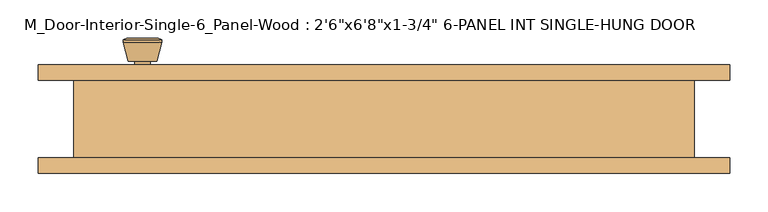
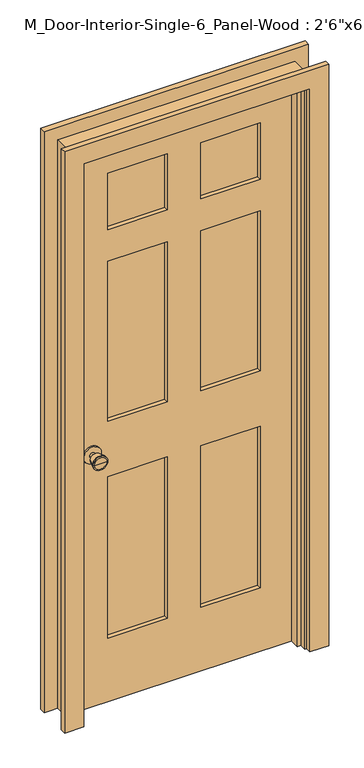
"""IFC4 building model written with IfcOpenShell, lengths in millimetres: door geometry."""

import ifcopenshell
import ifcopenshell.guid

model = None  # the IFC model being written
_history = None  # IfcOwnerHistory: only IFC2X3 demands one
_inside = {}  # id of a spatial element -> (the spatial element, [elements in it])
_under = {}  # id of a project, library or spatial element -> (it, [spatial elements below it])
_declared = {}  # id of a project -> (the project, [libraries it declares])
_typed = {}  # id of a type object -> (the type object, [elements of that type])
_made_of = {}  # id of a material, layer set ... -> (it, [elements and type objects made of it])


def new_model(schema):
    """Start an empty IFC model of exactly this schema.

    Asked for "IFC4X3", IfcOpenShell would pick the latest addendum, in which some entities
    have other attributes; the version numbers below select the first issue.
    IFC2X3 requires an IfcOwnerHistory on every rooted entity: one is made here for all.
    """
    global model, _history
    if schema == "IFC4X3":
        model = ifcopenshell.file(schema_version=(4, 3, 0, 0))
    else:
        model = ifcopenshell.file(schema=schema)
    _inside.clear()
    _under.clear()
    _declared.clear()
    _typed.clear()
    _made_of.clear()
    _history = None
    if model.schema == "IFC2X3":
        org = make("IfcOrganization", Name="unknown")
        user = make(
            "IfcPersonAndOrganization",
            ThePerson=make("IfcPerson", FamilyName="unknown"),
            TheOrganization=org,
        )
        app = make(
            "IfcApplication",
            ApplicationDeveloper=org,
            Version="unknown",
            ApplicationFullName="unknown",
            ApplicationIdentifier="unknown",
        )
        _history = make(
            "IfcOwnerHistory",
            OwningUser=user,
            OwningApplication=app,
            ChangeAction="ADDED",
            CreationDate=0,
        )
    return model


def make(cls, **values):
    """One entity of the class cls with the attributes given. An attribute that is None is left unset."""
    return model.create_entity(
        cls, **{name: value for name, value in values.items() if value is not None}
    )


def rooted(cls, **values):
    """An entity with a GlobalId (a new one), such as an element, a storey or a relation."""
    return make(cls, GlobalId=ifcopenshell.guid.new(), OwnerHistory=_history, **values)


def si_unit(unit_type, name, prefix=None):
    """IfcSIUnit, for example si_unit("LENGTHUNIT", "METRE", prefix="MILLI")."""
    return make("IfcSIUnit", UnitType=unit_type, Prefix=prefix, Name=name)


def assignment(units):
    """IfcUnitAssignment: the units of a project."""
    return None if units is None else make("IfcUnitAssignment", Units=units)


def point(xyz):
    """IfcCartesianPoint."""
    return None if xyz is None else make("IfcCartesianPoint", Coordinates=xyz)


def direction(xyz):
    """IfcDirection."""
    return None if xyz is None else make("IfcDirection", DirectionRatios=xyz)


def frame(location, z_axis=None, x_axis=None):
    """IfcAxis2Placement3D, a coordinate frame: its origin and axes. An axis left out is left unset."""
    return make(
        "IfcAxis2Placement3D",
        Location=point(location),
        Axis=direction(z_axis),
        RefDirection=direction(x_axis),
    )


def frame_2d(location, x_axis=None):
    """IfcAxis2Placement2D, a coordinate frame in the plane: its origin and x axis."""
    return make(
        "IfcAxis2Placement2D", Location=point(location), RefDirection=direction(x_axis)
    )


def origin():
    """The frame at (0, 0, 0) with its axes left unset."""
    return frame((0.0, 0.0, 0.0))


def place(relative_to, where):
    """IfcLocalPlacement: puts the frame where relative to a parent placement (None: the world)."""
    return make(
        "IfcLocalPlacement", PlacementRelTo=relative_to, RelativePlacement=where
    )


def context(
    kind, dimensions, precision=None, world=None, true_north=None, identifier=None
):
    """IfcGeometricRepresentationContext, for example the 3D "Model" context."""
    return make(
        "IfcGeometricRepresentationContext",
        ContextIdentifier=identifier,
        ContextType=kind,
        CoordinateSpaceDimension=dimensions,
        Precision=precision,
        WorldCoordinateSystem=world,
        TrueNorth=true_north,
    )


def project(units=None, contexts=None):
    """IfcProject with its units and contexts."""
    return rooted(
        "IfcProject",
        Name="project",
        RepresentationContexts=contexts,
        UnitsInContext=assignment(units),
    )


def spatial(cls, under=None, at=None, **own):
    """A site, building, storey or space (cls), placed at a placement, below another one or the project."""
    s = rooted(cls, ObjectPlacement=at, **own)
    if under is not None:
        _under.setdefault(under.id(), (under, []))[1].append(s)
    return s


def polyline(points):
    """IfcPolyline through the points."""
    return make("IfcPolyline", Points=[point(p) for p in points])


def circle_curve(where, radius):
    """IfcCircle in the frame where."""
    return make("IfcCircle", Position=where, Radius=radius)


def trimmed(basis, trim1, trim2, sense, master):
    """IfcTrimmedCurve: the piece of a basis curve between two trims."""
    return make(
        "IfcTrimmedCurve",
        BasisCurve=basis,
        Trim1=trim1,
        Trim2=trim2,
        SenseAgreement=sense,
        MasterRepresentation=master,
    )


def segment(curve, same_sense, transition):
    """IfcCompositeCurveSegment."""
    return make(
        "IfcCompositeCurveSegment",
        Transition=transition,
        SameSense=same_sense,
        ParentCurve=curve,
    )


def composite_curve(segments, self_intersect=None):
    """IfcCompositeCurve: segments joined end to end."""
    return make("IfcCompositeCurve", Segments=segments, SelfIntersect=self_intersect)


def outline(outer, holes=None, kind="AREA"):
    """IfcArbitraryClosedProfileDef: a profile drawn as a closed curve; with holes, ...WithVoids."""
    if holes is None:
        return make("IfcArbitraryClosedProfileDef", ProfileType=kind, OuterCurve=outer)
    return make(
        "IfcArbitraryProfileDefWithVoids",
        ProfileType=kind,
        OuterCurve=outer,
        InnerCurves=holes,
    )


def extrude(swept, where, along, depth):
    """IfcExtrudedAreaSolid: the profile swept, set in the frame where, extruded along a direction by depth."""
    return make(
        "IfcExtrudedAreaSolid",
        SweptArea=swept,
        Position=where,
        ExtrudedDirection=direction(along),
        Depth=depth,
    )


def faces_of(points, faces, orient=None, outer=None):
    """IfcFace entities. A face is a list of loops; a loop is a list of indices into points, from 0.

    orient and outer hold one flag for each loop. By default every Orientation is true, the
    first loop of a face is its IfcFaceOuterBound and the others are IfcFaceBound.
    """
    made = []
    for i, loops in enumerate(faces):
        bounds = []
        for j, loop in enumerate(loops):
            is_outer = j == 0 if outer is None else outer[i][j]
            bounds.append(
                make(
                    "IfcFaceOuterBound" if is_outer else "IfcFaceBound",
                    Bound=make("IfcPolyLoop", Polygon=[points[k] for k in loop]),
                    Orientation=True if orient is None else orient[i][j],
                )
            )
        made.append(make("IfcFace", Bounds=bounds))
    return made


def faceted_brep(points, faces, orient=None, outer=None, voids=None):
    """IfcFacetedBrep: a solid bounded by flat faces; with voids (closed shells), ...WithVoids."""
    shared = [point(p) for p in points]
    hull = make("IfcClosedShell", CfsFaces=faces_of(shared, faces, orient, outer))
    if voids is None:
        return make("IfcFacetedBrep", Outer=hull)
    return make(
        "IfcFacetedBrepWithVoids",
        Outer=hull,
        Voids=[
            make(cls, CfsFaces=faces_of(shared, fs, o, b)) for cls, fs, o, b in voids
        ],
    )


def shape(context_of_items, identifier, shape_type, items):
    """IfcShapeRepresentation: the items that make up one representation, for example the "Body"."""
    return make(
        "IfcShapeRepresentation",
        ContextOfItems=context_of_items,
        RepresentationIdentifier=identifier,
        RepresentationType=shape_type,
        Items=items,
    )


def source(mapping_origin, context_of_items, identifier, shape_type, items):
    """IfcRepresentationMap: a shape defined once, which mapped items show again and again."""
    return make(
        "IfcRepresentationMap",
        MappingOrigin=mapping_origin,
        MappedRepresentation=shape(context_of_items, identifier, shape_type, items),
    )


def transform(
    local_origin,
    x_axis=None,
    y_axis=None,
    z_axis=None,
    scale=None,
    scale2=None,
    scale3=None,
    uniform=True,
):
    """IfcCartesianTransformationOperator3D, or its non-uniform kind. x_axis, y_axis, z_axis: its Axis1, 2, 3."""
    if uniform:
        return make(
            "IfcCartesianTransformationOperator3D",
            Axis1=direction(x_axis),
            Axis2=direction(y_axis),
            LocalOrigin=point(local_origin),
            Scale=scale,
            Axis3=direction(z_axis),
        )
    return make(
        "IfcCartesianTransformationOperator3DnonUniform",
        Axis1=direction(x_axis),
        Axis2=direction(y_axis),
        LocalOrigin=point(local_origin),
        Scale=scale,
        Axis3=direction(z_axis),
        Scale2=scale2,
        Scale3=scale3,
    )


def mapped(mapping_source, mapping_target):
    """IfcMappedItem: shows the shape of a source again, moved by a transform."""
    return make(
        "IfcMappedItem", MappingSource=mapping_source, MappingTarget=mapping_target
    )


def made_of(thing, what):
    """Note that an element or type object is made of a material, layer set ...; save() writes the relation."""
    if what is not None:
        _made_of.setdefault(what.id(), (what, []))[1].append(thing)
    return thing


def element(
    cls,
    number,
    at=None,
    inside=None,
    cuts=None,
    type_object=None,
    material=None,
    context=None,
    identifier="Body",
    shape_type=None,
    held_by="IfcProductDefinitionShape",
    body=None,
    shapes=None,
    **own,
):
    """One element of the class cls, such as IfcWall. Its Tag is "e" and its number.

    at: its placement. inside: the storey or other place that contains it. cuts: it is an
    opening in that element (IfcRelVoidsElement). A single representation is given by context,
    identifier, shape_type and body (its items); several are given by shapes. held_by: the class
    of the entity that holds the representations. save() writes the other relations.
    """
    e = rooted(cls, Tag="e%d" % number, ObjectPlacement=at, **own)
    if body is not None:
        shapes = [shape(context, identifier, shape_type, body)]
    if shapes is not None:
        e.Representation = make(held_by, Representations=shapes)
    if inside is not None:
        _inside.setdefault(inside.id(), (inside, []))[1].append(e)
    if cuts is not None:
        rooted(
            "IfcRelVoidsElement", RelatingBuildingElement=cuts, RelatedOpeningElement=e
        )
    if type_object is not None:
        _typed.setdefault(type_object.id(), (type_object, []))[1].append(e)
    return made_of(e, material)


def aggregate(whole, parts):
    """IfcRelAggregates: a whole, such as a stair, and the parts it consists of."""
    return rooted("IfcRelAggregates", RelatingObject=whole, RelatedObjects=parts)


def save(model, path):
    """Write the relations noted so far, then the file.

    IfcRelAggregates (storeys below a building ...), IfcRelContainedInSpatialStructure (elements
    in a storey), IfcRelDefinesByType, IfcRelAssociatesMaterial and IfcRelDeclares: one each for
    every whole, place, type object, material and project.
    """
    for whole, parts in _under.values():
        aggregate(whole, parts)
    for where, things in _inside.values():
        rooted(
            "IfcRelContainedInSpatialStructure",
            RelatedElements=things,
            RelatingStructure=where,
        )
    for kind, things in _typed.values():
        rooted("IfcRelDefinesByType", RelatedObjects=things, RelatingType=kind)
    for what, things in _made_of.values():
        rooted("IfcRelAssociatesMaterial", RelatedObjects=things, RelatingMaterial=what)
    for by, libraries in _declared.values():
        rooted("IfcRelDeclares", RelatingContext=by, RelatedDefinitions=libraries)
    model.write(path)


def plane_surface(at):
    """IfcPlane: the flat surface through the origin of the frame at, square to its z axis."""
    return make("IfcPlane", Position=at)


def cylinder_surface(at, radius):
    """IfcCylindricalSurface: all points at the distance radius from the z axis of the frame at."""
    return make("IfcCylindricalSurface", Position=at, Radius=radius)


def revolved_surface(curve, axis_point, axis_direction):
    """IfcSurfaceOfRevolution: the curve turned about the line through axis_point along axis_direction."""
    return make(
        "IfcSurfaceOfRevolution",
        SweptCurve=make("IfcArbitraryOpenProfileDef", ProfileType="CURVE", Curve=curve),
        AxisPosition=make("IfcAxis1Placement", Location=point(axis_point), Axis=direction(axis_direction)),
    )


def advanced_brep(points, edges, surfaces, faces):
    """IfcAdvancedBrep: a solid bounded by faces that lie on surfaces and meet in shared edges.

    An edge is (start, end): straight between two places in points (the first is 0);
    or (start, end, curve); or (start, end, curve, False) where it runs against its curve.
    A face is (place in surfaces, loops), or (place, loops, False) where it looks against
    its surface's normal. A loop lists edges by number (the first is 1), with a minus sign
    where the edge is run from its end to its start. The first loop is the outer one.
    """
    corners = [point(p) for p in points]
    vertices = [make("IfcVertexPoint", VertexGeometry=c) for c in corners]
    made = []
    for start, end, *more in edges:
        made.append(
            make(
                "IfcEdgeCurve",
                EdgeStart=vertices[start],
                EdgeEnd=vertices[end],
                EdgeGeometry=more[0] if more else make("IfcPolyline", Points=[corners[start], corners[end]]),
                SameSense=more[1] if len(more) > 1 else True,
            )
        )
    hull = []
    for where, loops, *sense in faces:
        bounds = []
        for j, loop in enumerate(loops):
            ring = [make("IfcOrientedEdge", EdgeElement=made[abs(k) - 1], Orientation=k > 0) for k in loop]
            bounds.append(
                make(
                    "IfcFaceOuterBound" if j == 0 else "IfcFaceBound",
                    Bound=make("IfcEdgeLoop", EdgeList=ring),
                    Orientation=True,
                )
            )
        hull.append(make("IfcAdvancedFace", Bounds=bounds, FaceSurface=surfaces[where], SameSense=sense[0] if sense else True))
    return make("IfcAdvancedBrep", Outer=make("IfcClosedShell", CfsFaces=hull))


def door_beb2e203(model_context):
    return source(origin(), model_context, "Body", "SolidModel", [
        advanced_brep(
        [(-316.0, -2.825, 914.4), (-306.0, -2.825, 914.4), (-326.0, -2.825, 914.4), (-295.5241324, -51.825, 914.4), (-316.0, -51.825, 914.4), (-336.4758676, -51.825, 914.4), (-291.0, -49.9971319, 914.4), (-341.0, -49.9971319, 914.4), (-291.0, -46.5334537, 914.4), (-341.0, -46.5334537, 914.4), (-297.363764, -21.825, 914.4), (-334.636236, -21.825, 914.4), (-306.0, -21.825, 914.4), (-326.0, -21.825, 914.4)],
        [
            (0, 1),
            (1, 2, circle_curve(frame((-316.0, -2.825, 914.4), z_axis=(0.0, 1.0, 0.0), x_axis=(-1.0, 0.0, 0.0)), 10.0)),
            (2, 0),
            (2, 1, circle_curve(frame((-316.0, -2.825, 914.4), z_axis=(0.0, 1.0, 0.0), x_axis=(-1.0, 0.0, 0.0)), 10.0)),
            (3, 4),
            (4, 5),
            (5, 3, circle_curve(frame((-316.0, -51.825, 914.4), z_axis=(0.0, -1.0, 0.0), x_axis=(-1.0, 0.0, 0.0)), 20.4758676)),
            (3, 5, circle_curve(frame((-316.0, -51.825, 914.4), z_axis=(0.0, -1.0, 0.0), x_axis=(-1.0, 0.0, 0.0)), 20.4758676)),
            (6, 3),
            (5, 7),
            (7, 6, circle_curve(frame((-316.0, -49.9971319, 914.4), z_axis=(0.0, -1.0, 0.0), x_axis=(-1.0, 0.0, 0.0)), 25.0)),
            (6, 7, circle_curve(frame((-316.0, -49.9971319, 914.4), z_axis=(0.0, -1.0, 0.0), x_axis=(-1.0, 0.0, 0.0)), 25.0)),
            (8, 6),
            (7, 9),
            (9, 8, circle_curve(frame((-316.0, -46.5334537, 914.4), z_axis=(0.0, -1.0, 0.0), x_axis=(-1.0, 0.0, 0.0)), 25.0)),
            (8, 9, circle_curve(frame((-316.0, -46.5334537, 914.4), z_axis=(0.0, -1.0, 0.0), x_axis=(-1.0, 0.0, 0.0)), 25.0)),
            (10, 8),
            (9, 11),
            (11, 10, circle_curve(frame((-316.0, -21.825, 914.4), z_axis=(0.0, -1.0, 0.0), x_axis=(-1.0, 0.0, 0.0)), 18.636236)),
            (10, 11, circle_curve(frame((-316.0, -21.825, 914.4), z_axis=(0.0, -1.0, 0.0), x_axis=(-1.0, 0.0, 0.0)), 18.636236)),
            (12, 10),
            (11, 13),
            (13, 12, circle_curve(frame((-316.0, -21.825, 914.4), z_axis=(0.0, -1.0, 0.0), x_axis=(-1.0, 0.0, 0.0)), 10.0)),
            (12, 13, circle_curve(frame((-316.0, -21.825, 914.4), z_axis=(0.0, -1.0, 0.0), x_axis=(-1.0, 0.0, 0.0)), 10.0)),
            (1, 12),
            (13, 2),
        ],
        [
            plane_surface(frame((-316.0, -2.825, 914.4), z_axis=(0.0, 1.0, 0.0), x_axis=(-1.0, 0.0, 0.0))),
            plane_surface(frame((-316.0, -51.825, 914.4), z_axis=(0.0, -1.0, 0.0), x_axis=(-1.0, 0.0, 0.0))),
            revolved_surface(polyline([(-336.4758676, -51.825, 914.4), (-341.0, -49.9971319, 914.4)]), (-316.0, -2.825, 914.4), (0.0, 1.0, 0.0)),
            cylinder_surface(frame((-316.0, -2.825, 914.4), z_axis=(0.0, 1.0, 0.0), x_axis=(-1.0, 0.0, 0.0)), 25.0),
            revolved_surface(polyline([(-341.0, -46.5334537, 914.4), (-334.636236, -21.825, 914.4)]), (-316.0, -2.825, 914.4), (0.0, 1.0, 0.0)),
            plane_surface(frame((-316.0, -21.825, 914.4), z_axis=(0.0, 1.0, 0.0), x_axis=(-1.0, 0.0, 0.0))),
            cylinder_surface(frame((-316.0, -2.825, 914.4), z_axis=(0.0, 1.0, 0.0), x_axis=(-1.0, 0.0, 0.0)), 10.0),
        ],
        [
            (0, [[1, 2, 3]]),
            (0, [[-3, 4, -1]]),
            (1, [[5, 6, 7]]),
            (1, [[-6, -5, 8]]),
            (2, [[9, -7, 10, 11]]),
            (2, [[-10, -8, -9, 12]]),
            (3, [[13, -11, 14, 15]]),
            (3, [[-14, -12, -13, 16]]),
            (4, [[17, -15, 18, 19]]),
            (4, [[-18, -16, -17, 20]]),
            (5, [[21, -19, 22, 23]]),
            (5, [[-22, -20, -21, 24]]),
            (6, [[25, -23, 26, -2]]),
            (6, [[-26, -24, -25, -4]]),
        ],
    ),
        extrude(outline(composite_curve([segment(trimmed(circle_curve(frame_2d((914.4, -316.0)), 30.0), [point((914.4, -346.0))], [point((914.4, -286.0))], False, "CARTESIAN"), True, "CONTINUOUS"), segment(trimmed(circle_curve(frame_2d((914.4, -316.0)), 30.0), [point((914.4, -286.0))], [point((914.4, -346.0))], False, "CARTESIAN"), True, "CONTINUOUS")], self_intersect=False)), frame((0.0, -2.825, 0.0), z_axis=(0.0, 1.0, 0.0), x_axis=(0.0, 0.0, 1.0)), (0.0, 0.0, 1.0), 6.0),
        advanced_brep(
        [(-316.0, 53.625, 914.4), (-326.0, 53.625, 914.4), (-306.0, 53.625, 914.4), (-295.5241324, 102.625, 914.4), (-336.4758676, 102.625, 914.4), (-316.0, 102.625, 914.4), (-291.0, 100.7971319, 914.4), (-341.0, 100.7971319, 914.4), (-291.0, 97.3334537, 914.4), (-341.0, 97.3334537, 914.4), (-297.363764, 72.625, 914.4), (-334.636236, 72.625, 914.4), (-306.0, 72.625, 914.4), (-326.0, 72.625, 914.4)],
        [
            (0, 1),
            (1, 2, circle_curve(frame((-316.0, 53.625, 914.4), z_axis=(0.0, -1.0, 0.0), x_axis=(-1.0, 0.0, 0.0)), 10.0)),
            (2, 0),
            (2, 1, circle_curve(frame((-316.0, 53.625, 914.4), z_axis=(0.0, -1.0, 0.0), x_axis=(-1.0, 0.0, 0.0)), 10.0)),
            (3, 4, circle_curve(frame((-316.0, 102.625, 914.4), z_axis=(0.0, 1.0, 0.0), x_axis=(-1.0, 0.0, 0.0)), 20.4758676)),
            (4, 5),
            (5, 3),
            (4, 3, circle_curve(frame((-316.0, 102.625, 914.4), z_axis=(0.0, 1.0, 0.0), x_axis=(-1.0, 0.0, 0.0)), 20.4758676)),
            (6, 7, circle_curve(frame((-316.0, 100.7971319, 914.4), z_axis=(0.0, 1.0, 0.0), x_axis=(-1.0, 0.0, 0.0)), 25.0)),
            (7, 4),
            (3, 6),
            (7, 6, circle_curve(frame((-316.0, 100.7971319, 914.4), z_axis=(0.0, 1.0, 0.0), x_axis=(-1.0, 0.0, 0.0)), 25.0)),
            (8, 9, circle_curve(frame((-316.0, 97.3334537, 914.4), z_axis=(0.0, 1.0, 0.0), x_axis=(-1.0, 0.0, 0.0)), 25.0)),
            (9, 7),
            (6, 8),
            (9, 8, circle_curve(frame((-316.0, 97.3334537, 914.4), z_axis=(0.0, 1.0, 0.0), x_axis=(-1.0, 0.0, 0.0)), 25.0)),
            (10, 11, circle_curve(frame((-316.0, 72.625, 914.4), z_axis=(0.0, 1.0, 0.0), x_axis=(-1.0, 0.0, 0.0)), 18.636236)),
            (11, 9),
            (8, 10),
            (11, 10, circle_curve(frame((-316.0, 72.625, 914.4), z_axis=(0.0, 1.0, 0.0), x_axis=(-1.0, 0.0, 0.0)), 18.636236)),
            (12, 13, circle_curve(frame((-316.0, 72.625, 914.4), z_axis=(0.0, 1.0, 0.0), x_axis=(-1.0, 0.0, 0.0)), 10.0)),
            (13, 11),
            (10, 12),
            (13, 12, circle_curve(frame((-316.0, 72.625, 914.4), z_axis=(0.0, 1.0, 0.0), x_axis=(-1.0, 0.0, 0.0)), 10.0)),
            (1, 13),
            (12, 2),
        ],
        [
            plane_surface(frame((-316.0, 53.625, 914.4), z_axis=(0.0, -1.0, 0.0), x_axis=(-1.0, 0.0, 0.0))),
            plane_surface(frame((-316.0, 102.625, 914.4), z_axis=(0.0, 1.0, 0.0), x_axis=(-1.0, 0.0, 0.0))),
            revolved_surface(polyline([(-336.4758676, 102.625, 914.4), (-341.0, 100.7971319, 914.4)]), (-316.0, 53.625, 914.4), (0.0, -1.0, 0.0)),
            cylinder_surface(frame((-316.0, 53.625, 914.4), z_axis=(0.0, -1.0, 0.0), x_axis=(-1.0, 0.0, 0.0)), 25.0),
            revolved_surface(polyline([(-341.0, 97.3334537, 914.4), (-334.636236, 72.625, 914.4)]), (-316.0, 53.625, 914.4), (0.0, -1.0, 0.0)),
            plane_surface(frame((-316.0, 72.625, 914.4), z_axis=(0.0, -1.0, 0.0), x_axis=(-1.0, 0.0, 0.0))),
            cylinder_surface(frame((-316.0, 53.625, 914.4), z_axis=(0.0, -1.0, 0.0), x_axis=(-1.0, 0.0, 0.0)), 10.0),
        ],
        [
            (0, [[1, 2, 3]]),
            (0, [[-3, 4, -1]]),
            (1, [[5, 6, 7]]),
            (1, [[8, -7, -6]]),
            (2, [[9, 10, -5, 11]]),
            (2, [[12, -11, -8, -10]]),
            (3, [[13, 14, -9, 15]]),
            (3, [[16, -15, -12, -14]]),
            (4, [[17, 18, -13, 19]]),
            (4, [[20, -19, -16, -18]]),
            (5, [[21, 22, -17, 23]]),
            (5, [[24, -23, -20, -22]]),
            (6, [[-2, 25, -21, 26]]),
            (6, [[-4, -26, -24, -25]]),
        ],
    ),
        extrude(outline(composite_curve([segment(trimmed(circle_curve(frame_2d((914.4, -316.0)), 30.0), [point((914.4, -346.0))], [point((914.4, -286.0))], False, "CARTESIAN"), True, "CONTINUOUS"), segment(trimmed(circle_curve(frame_2d((914.4, -316.0)), 30.0), [point((914.4, -286.0))], [point((914.4, -346.0))], False, "CARTESIAN"), True, "CONTINUOUS")], self_intersect=False)), frame((0.0, 47.625, 0.0), z_axis=(0.0, 1.0, 0.0), x_axis=(0.0, 0.0, 1.0)), (0.0, 0.0, 1.0), 6.0),
        extrude(outline(polyline([(261.0, 17.9916667), (57.5, 17.9916667), (57.5, 32.8083333), (261.0, 32.8083333), (261.0, 17.9916667)])), frame((0.0, 0.0, 1708.5), z_axis=(0.0, 0.0, 1.0), x_axis=(1.0, 0.0, 0.0)), (0.0, 0.0, 1.0), 203.5),
        extrude(outline(polyline([(261.0, 17.9916667), (57.5, 17.9916667), (57.5, 32.8083333), (261.0, 32.8083333), (261.0, 17.9916667)])), frame((0.0, 0.0, 1014.4), z_axis=(0.0, 0.0, 1.0), x_axis=(1.0, 0.0, 0.0)), (0.0, 0.0, 1.0), 579.1),
        extrude(outline(polyline([(-57.5, 17.9916667), (-261.0, 17.9916667), (-261.0, 32.8083333), (-57.5, 32.8083333), (-57.5, 17.9916667)])), frame((0.0, 0.0, 1014.4), z_axis=(0.0, 0.0, 1.0), x_axis=(1.0, 0.0, 0.0)), (0.0, 0.0, 1.0), 579.1),
        extrude(outline(polyline([(-57.5, 17.9916667), (-261.0, 17.9916667), (-261.0, 32.8083333), (-57.5, 32.8083333), (-57.5, 17.9916667)])), frame((0.0, 0.0, 1708.5), z_axis=(0.0, 0.0, 1.0), x_axis=(1.0, 0.0, 0.0)), (0.0, 0.0, 1.0), 203.5),
        extrude(outline(polyline([(261.0, 17.9916667), (57.5, 17.9916667), (57.5, 32.8083333), (261.0, 32.8083333), (261.0, 17.9916667)])), frame((0.0, 0.0, 230.0), z_axis=(0.0, 0.0, 1.0), x_axis=(1.0, 0.0, 0.0)), (0.0, 0.0, 1.0), 584.4),
        extrude(outline(polyline([(-57.5, 17.9916667), (-261.0, 17.9916667), (-261.0, 32.8083333), (-57.5, 32.8083333), (-57.5, 17.9916667)])), frame((0.0, 0.0, 230.0), z_axis=(0.0, 0.0, 1.0), x_axis=(1.0, 0.0, 0.0)), (0.0, 0.0, 1.0), 584.4),
        extrude(outline(polyline([(2032.0, -381.0), (0.0, -381.0), (0.0, 381.0), (2032.0, 381.0), (2032.0, -381.0)]), holes=[polyline([(1912.0, 57.5), (1912.0, 261.0), (1708.5, 261.0), (1708.5, 57.5), (1912.0, 57.5)]), polyline([(1593.5, 261.0), (1014.4, 261.0), (1014.4, 57.5), (1593.5, 57.5), (1593.5, 261.0)]), polyline([(1014.4, -57.5), (1014.4, -261.0), (1593.5, -261.0), (1593.5, -57.5), (1014.4, -57.5)]), polyline([(1708.5, -261.0), (1912.0, -261.0), (1912.0, -57.5), (1708.5, -57.5), (1708.5, -261.0)]), polyline([(814.4, 57.5), (814.4, 261.0), (230.0, 261.0), (230.0, 57.5), (814.4, 57.5)]), polyline([(230.0, -57.5), (230.0, -261.0), (814.4, -261.0), (814.4, -57.5), (230.0, -57.5)])]), frame((0.0, 3.175, 0.0), z_axis=(0.0, 1.0, 0.0), x_axis=(0.0, 0.0, 1.0)), (0.0, 0.0, 1.0), 44.45),
        faceted_brep([(406.0, 47.625, 0.0), (406.0, -53.975, 0.0), (381.0, -53.975, 0.0), (381.0, -31.75, 0.0), (368.3, -31.75, 0.0), (368.3, 3.175, 0.0), (381.0, 3.175, 0.0), (381.0, 47.625, 0.0), (406.0, 47.625, 2057.0), (406.0, -53.975, 2057.0), (-406.0, -53.975, 2057.0), (-406.0, -53.975, 0.0), (-381.0, -53.975, 0.0), (-381.0, -53.975, 2032.0), (381.0, -53.975, 2032.0), (381.0, -31.75, 2032.0), (-381.0, -31.75, 2032.0), (-381.0, -31.75, 0.0), (-368.3, -31.75, 0.0), (-368.3, -31.75, 2019.3), (368.3, -31.75, 2019.3), (368.3, 3.175, 2019.3), (-368.3, 3.175, 2019.3), (-368.3, 3.175, 0.0), (-381.0, 3.175, 0.0), (-381.0, 3.175, 2032.0), (381.0, 3.175, 2032.0), (381.0, 47.625, 2032.0), (-381.0, 47.625, 2032.0), (-381.0, 47.625, 0.0), (-406.0, 47.625, 0.0), (-406.0, 47.625, 2057.0)], [[[0, 1, 2, 3, 4, 5, 6, 7]], [[1, 0, 8, 9]], [[2, 1, 9, 10, 11, 12, 13, 14]], [[3, 2, 14, 15]], [[4, 3, 15, 16, 17, 18, 19, 20]], [[5, 4, 20, 21]], [[6, 5, 21, 22, 23, 24, 25, 26]], [[7, 6, 26, 27]], [[0, 7, 27, 28, 29, 30, 31, 8]], [[9, 8, 31, 10]], [[15, 14, 13, 16]], [[21, 20, 19, 22]], [[27, 26, 25, 28]], [[30, 29, 24, 23, 18, 17, 12, 11]], [[10, 31, 30, 11]], [[16, 13, 12, 17]], [[22, 19, 18, 23]], [[28, 25, 24, 29]]]),
        extrude(outline(polyline([(0.0, 387.35), (0.0, 452.35), (2103.35, 452.35), (2103.35, -452.35), (0.0, -452.35), (0.0, -387.35), (2038.35, -387.35), (2038.35, 387.35), (0.0, 387.35)])), frame((0.0, -73.975, 0.0), z_axis=(0.0, 1.0, 0.0), x_axis=(0.0, 0.0, 1.0)), (0.0, 0.0, 1.0), 20.0),
        extrude(outline(polyline([(0.0, 387.35), (0.0, 452.35), (2103.35, 452.35), (2103.35, -452.35), (0.0, -452.35), (0.0, -387.35), (2038.35, -387.35), (2038.35, 387.35), (0.0, 387.35)])), frame((0.0, 47.625, 0.0), z_axis=(0.0, 1.0, 0.0), x_axis=(0.0, 0.0, 1.0)), (0.0, 0.0, 1.0), 20.0),
    ])


if __name__ == "__main__":
    model = new_model("IFC4")
    model_context = context("Model", 3, world=origin())
    ifc_project = project(units=[si_unit("LENGTHUNIT", "METRE", prefix="MILLI")], contexts=[model_context])
    site = spatial("IfcSite", under=ifc_project)
    building = spatial("IfcBuilding", under=site)
    placement = place(None, origin())
    door_shape = door_beb2e203(model_context)
    element("IfcDoor", 1, ObjectType="M_Door-Interior-Single-6_Panel-Wood : 2'6\"x6'8\"x1-3/4\" 6-PANEL INT SINGLE-HUNG DOOR", at=placement, inside=building, context=model_context, shape_type="MappedRepresentation", body=[
        mapped(door_shape, transform((0.0, 0.0, 0.0), x_axis=(1.0, 0.0, 0.0), y_axis=(0.0, 1.0, 0.0), z_axis=(0.0, 0.0, 1.0))),
    ])
    save(model, "model.ifc")

# Revit data of these elements
# Type "M_Door-Interior-Single-6_Panel-Wood : 2'6\"x6'8\"x1-3/4\" 6-PANEL INT SINGLE-HUNG DOOR"
#   Type Mark = "11"
#   Assembly Code = "C1020300"
#   Analytic Construction = "Wooden"
#   Top Rail = 0' - 4.72441"
#   Top Panel = 0' - 8.01181"
#   Thickness = 0' - 1 3/4"
#   Thermal Resistance (R) = 2.5876 (h·ft²·°F)/BTU
#   Swing Angle [instance default] = 90.00°
#   Stiles = 0' - 4.72441"
#   Rough Width = 2' - 7.9685"
#   Rough Height = 6' - 8.98425"
#   Mullion = 0' - 4.52756"
#   Lock Rail = 0' - 7.87402"
#   Intermediate Rail = 0' - 4.52756"
#   Height = 6' - 8"
#   Width = 2' - 6"
#   Heat Transfer Coefficient (U) = 0.3865 BTU/(h·ft²·°F)
#   Bottom Rail = 0' - 9.05512"
#   Trim Material = Cherry
#   Panel Material = Cherry
#   Frame Material = Cherry
#   Door Handle Material = Aluminum
#   Visual Light Transmittance = 0
#   Solar Heat Gain Coefficient = 0
#   Wall Closure = (empty or 0)
#   Function = (empty or 0)
# Element 1 (IfcDoor, "M_Door-Interior-Single-6_Panel-Wood : 2'6\"x6'8\"x1-3/4\" 6-PANEL INT SINGLE-HUNG DOOR")
#   Materials on its faces: "Cherry", "Aluminum"
# Materials
#   "Cherry": class "Wood", colour RGB 226 177 128, transparency 0, Description = "Prunus Serotina", Cost = 0
#   "Aluminum": class "Metal", colour RGB 244 244 244, transparency 0, Description = "Aluminum 6061", Cost = 0
